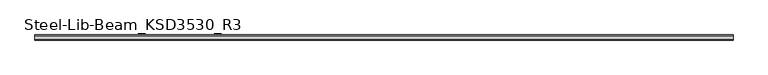
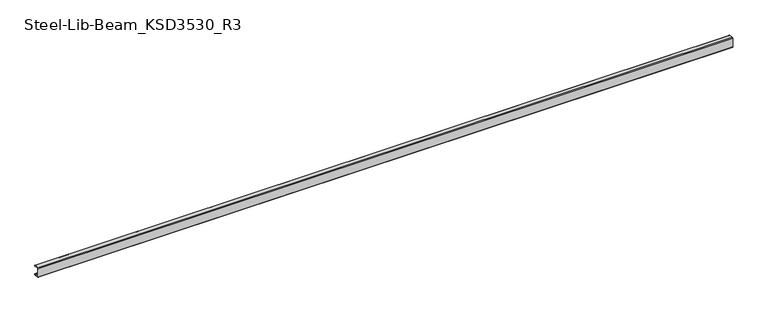
"""IFC4 building model written with IfcOpenShell, lengths in millimetres: beam geometry, Steel-Lib-Beam_KSD3530_R3 : BMS291_C-150×75x20x4.5."""

from ifc_helpers import new_model, si_unit, point, frame, frame_2d, origin, place, context, project, spatial, polyline, circle_curve, trimmed, segment, composite_curve, outline, extrude, source, transform, mapped, element, save


def steel_lib_beam_ksd3530_r3_ae8bddfd(model_context):
    return source(origin(), model_context, "Body", "SweptSolid", [
        extrude(outline(composite_curve([segment(polyline([(50.0, 66.0), (50.0, 55.0), (45.5, 55.0), (45.5, 66.0)]), True, "CONTINUOUS"), segment(trimmed(circle_curve(frame_2d((41.0, 66.0)), 4.5), [point((45.5, 66.0))], [point((41.0, 70.5))], True, "CARTESIAN"), True, "CONTINUOUS"), segment(polyline([(41.0, 70.5), (-16.0, 70.5)]), True, "CONTINUOUS"), segment(trimmed(circle_curve(frame_2d((-16.0, 66.0)), 4.5), [point((-16.0, 70.5))], [point((-20.5, 66.0))], True, "CARTESIAN"), True, "CONTINUOUS"), segment(polyline([(-20.5, 66.0), (-20.5, -66.0)]), True, "CONTINUOUS"), segment(trimmed(circle_curve(frame_2d((-16.0, -66.0)), 4.5), [point((-20.5, -66.0))], [point((-16.0, -70.5))], True, "CARTESIAN"), True, "CONTINUOUS"), segment(polyline([(-16.0, -70.5), (41.0, -70.5)]), True, "CONTINUOUS"), segment(trimmed(circle_curve(frame_2d((41.0, -66.0)), 4.5), [point((41.0, -70.5))], [point((45.5, -66.0))], True, "CARTESIAN"), True, "CONTINUOUS"), segment(polyline([(45.5, -66.0), (45.5, -55.0), (50.0, -55.0), (50.0, -66.0)]), True, "CONTINUOUS"), segment(trimmed(circle_curve(frame_2d((41.0, -66.0)), 9.0), [point((50.0, -66.0))], [point((41.0, -75.0))], False, "CARTESIAN"), True, "CONTINUOUS"), segment(polyline([(41.0, -75.0), (-16.0, -75.0)]), True, "CONTINUOUS"), segment(trimmed(circle_curve(frame_2d((-16.0, -66.0)), 9.0), [point((-16.0, -75.0))], [point((-25.0, -66.0))], False, "CARTESIAN"), True, "CONTINUOUS"), segment(polyline([(-25.0, -66.0), (-25.0, 66.0)]), True, "CONTINUOUS"), segment(trimmed(circle_curve(frame_2d((-16.0, 66.0)), 9.0), [point((-25.0, 66.0))], [point((-16.0, 75.0))], False, "CARTESIAN"), True, "CONTINUOUS"), segment(polyline([(-16.0, 75.0), (41.0, 75.0)]), True, "CONTINUOUS"), segment(trimmed(circle_curve(frame_2d((41.0, 66.0)), 9.0), [point((41.0, 75.0))], [point((50.0, 66.0))], False, "CARTESIAN"), True, "CONTINUOUS")], self_intersect=False)), frame((-5049.5, 0.0, 0.0), z_axis=(1.0, 0.0, 0.0), x_axis=(0.0, 1.0, 0.0)), (0.0, 0.0, 1.0), 10224.0),
    ])


if __name__ == "__main__":
    model = new_model("IFC4")
    model_context = context("Model", 3, world=origin())
    ifc_project = project(units=[si_unit("LENGTHUNIT", "METRE", prefix="MILLI")], contexts=[model_context])
    site = spatial("IfcSite", under=ifc_project)
    building = spatial("IfcBuilding", under=site)
    placement = place(None, origin())
    steel_lib_beam_ksd3530_r3_shape = steel_lib_beam_ksd3530_r3_ae8bddfd(model_context)
    element("IfcBeam", 1, ObjectType="Steel-Lib-Beam_KSD3530_R3 : BMS291_C-150×75x20x4.5", at=placement, inside=building, context=model_context, shape_type="MappedRepresentation", body=[
        mapped(steel_lib_beam_ksd3530_r3_shape, transform((0.0, 0.0, 0.0), x_axis=(1.0, 0.0, 0.0), y_axis=(0.0, 1.0, 0.0), z_axis=(0.0, 0.0, 1.0))),
    ])
    save(model, "model.ifc")

# Revit data of these elements
# Type "Steel-Lib-Beam_KSD3530_R3 : BMS291_C-150×75x20x4.5"
#   Keynote = "C-150×75x20x4.5"
#   SteelWeight = "Light"
#   x = 0.0250 m
#   t1 = 0.0090 m
#   t = 0.0045 m
#   Surface Area = 0.629834 m²/m
#   Section Area = 13.9688 cm²
#   Mass per Unit Length = 10.9655 kg/m
#   C = 0.0200 m
#   A = 0.0750 m
#   Length [instance default] = 1.5000 m
#   H = 0.1500 m
#   hec_material4 [instance default] = none
#   hec_material3 [instance default] = none
#   hec_material2 [instance default] = none
#   hec_material1 [instance default] = none
#   Structural Material [instance default] = Metal - Steel - Light Gauge
#   Assembly Code = ""
# Element 1 (IfcBeam, "Steel-Lib-Beam_KSD3530_R3 : BMS291_C-150×75x20x4.5")
#   Structural Material = none
# Materials
#   "Metal - Steel - Light Gauge": class "Metal", colour RGB 247 247 247, transparency 0
